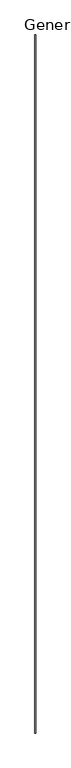
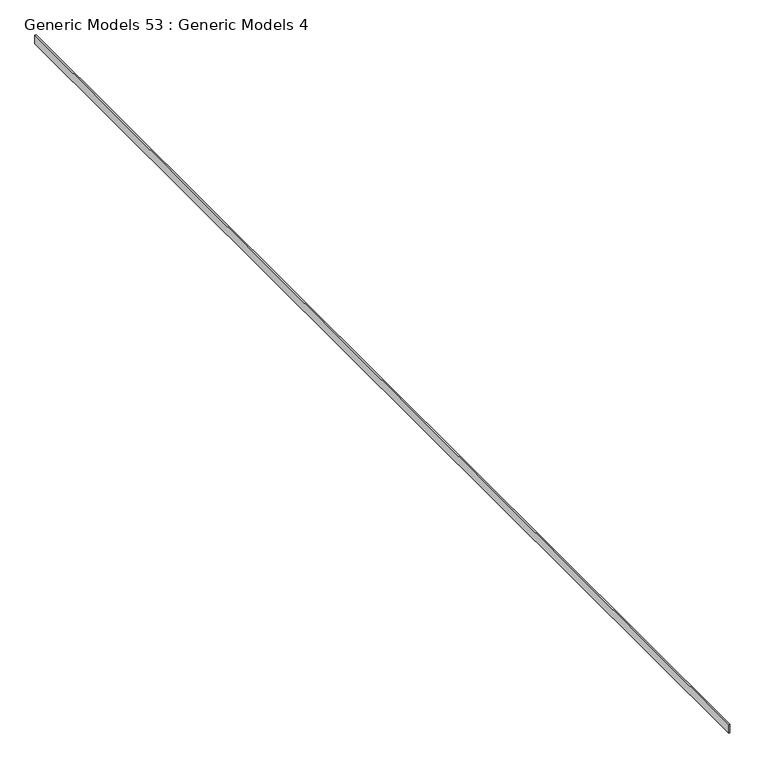
"""IFC4 building model written with IfcOpenShell, lengths in millimetres: proxy geometry, Generic Models 53 : Generic Models 4."""

from ifc_helpers import new_model, si_unit, frame, origin, place, context, project, spatial, polyline, outline, extrude, source, transform, mapped, element, save


def generic_models_53_generic_models_4_1300fac3(model_context):
    return source(origin(), model_context, "Body", "SweptSolid", [
        extrude(outline(polyline([(7253.8514146, -6864.9230338), (7234.8014146, -6864.9230338), (7234.8014146, 11778.6769662), (7253.8514146, 11778.6769662), (7253.8514146, -6864.9230338)])), frame((0.0, 0.0, 126778.6280968), z_axis=(0.0, 0.0, 1.0), x_axis=(1.0, 0.0, 0.0)), (0.0, 0.0, 1.0), 139.0309129),
    ])


if __name__ == "__main__":
    model = new_model("IFC4")
    model_context = context("Model", 3, world=origin())
    ifc_project = project(units=[si_unit("LENGTHUNIT", "METRE", prefix="MILLI")], contexts=[model_context])
    site = spatial("IfcSite", under=ifc_project)
    building = spatial("IfcBuilding", under=site)
    placement = place(None, origin())
    generic_models_53_generic_models_4_shape = generic_models_53_generic_models_4_1300fac3(model_context)
    element("IfcBuildingElementProxy", 1, Name="Generic Models 53 : Generic Models 4", ObjectType="Generic Models 53 : Generic Models 4", at=placement, inside=building, context=model_context, shape_type="MappedRepresentation", body=[
        mapped(generic_models_53_generic_models_4_shape, transform((0.0, 0.0, 0.0), x_axis=(1.0, 0.0, 0.0), y_axis=(0.0, 1.0, 0.0), z_axis=(0.0, 0.0, 1.0))),
    ])
    save(model, "model.ifc")

# Revit data of these elements
# Element 1 (IfcBuildingElementProxy, "Generic Models 53 : Generic Models 4")
#   Materials on its faces: "_CDX PLYWOOD - SEE STRUCT DWGs"
# Materials
#   "_CDX PLYWOOD - SEE STRUCT DWGs": class "Generic", colour RGB 98 75 74, transparency 0, Cost = 0
